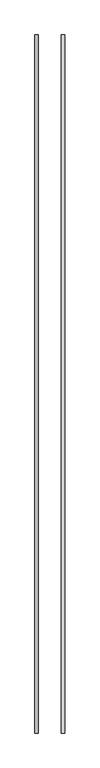
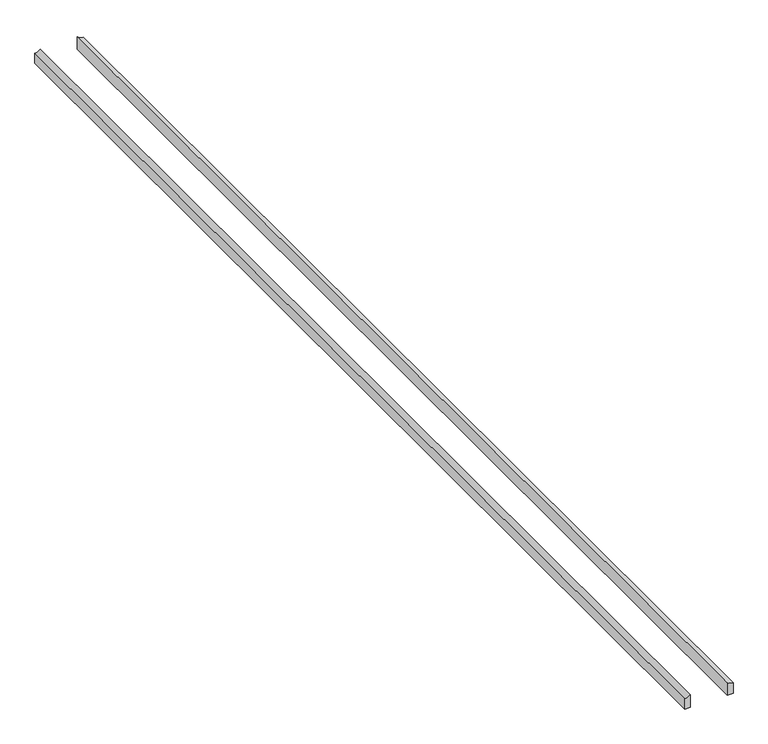
"""IFC4 building model written with IfcOpenShell, lengths in millimetres: proxy geometry, Joint027 17850 : Joint027 17850."""

from ifc_helpers import new_model, si_unit, point, frame, frame_2d, origin, place, context, project, spatial, polyline, circle_curve, trimmed, segment, composite_curve, outline, extrude, source, transform, mapped, element, save


def generic_models_950220de(model_context):
    return source(origin(), model_context, "Body", "SweptSolid", [
        extrude(outline(composite_curve([segment(polyline([(40150.796, 7291.9824219), (40131.746, 7291.9824219), (40131.746, 7301.4512927), (40155.1385809, 7301.4512927)]), True, "CONTINUOUS"), segment(trimmed(circle_curve(frame_2d((40161.3798693, 7292.8587095)), 10.6200833), [point((40155.1385809, 7301.4512927))], [point((40150.796, 7291.9824219))], True, "CARTESIAN"), True, "CONTINUOUS")], self_intersect=False)), frame((0.0, -3747.9491938, 0.0), z_axis=(0.0, 1.0, 0.0), x_axis=(0.0, 0.0, 1.0)), (0.0, 0.0, 1.0), 2000.0),
        extrude(outline(composite_curve([segment(trimmed(circle_curve(frame_2d((40167.1736286, 7377.7892228)), 16.1957742), [point((40150.9781799, 7377.6865442))], [point((40155.1385809, 7366.9512927))], True, "CARTESIAN"), True, "CONTINUOUS"), segment(polyline([(40155.1385809, 7366.9512927), (40131.746, 7366.9512927), (40131.746, 7377.6865442), (40150.9781799, 7377.6865442)]), True, "CONTINUOUS")], self_intersect=False)), frame((0.0, -3747.9491938, 0.0), z_axis=(0.0, 1.0, 0.0), x_axis=(0.0, 0.0, 1.0)), (0.0, 0.0, 1.0), 2000.0),
    ])


if __name__ == "__main__":
    model = new_model("IFC4")
    model_context = context("Model", 3, world=origin())
    ifc_project = project(units=[si_unit("LENGTHUNIT", "METRE", prefix="MILLI")], contexts=[model_context])
    site = spatial("IfcSite", under=ifc_project)
    building = spatial("IfcBuilding", under=site)
    placement = place(None, origin())
    generic_models_shape = generic_models_950220de(model_context)
    element("IfcBuildingElementProxy", 1, Name="Joint027 17850 : Joint027 17850", ObjectType="Joint027 17850 : Joint027 17850", at=placement, inside=building, context=model_context, shape_type="MappedRepresentation", body=[
        mapped(generic_models_shape, transform((0.0, 0.0, 0.0), x_axis=(1.0, 0.0, 0.0), y_axis=(0.0, 1.0, 0.0), z_axis=(0.0, 0.0, 1.0))),
    ])
    save(model, "model.ifc")

# Revit data of these elements
# Type "Joint027 17850 : Joint027 17850"
#   NameOverride = "Joint027"
# Element 1 (IfcBuildingElementProxy, "Joint027 17850 : Joint027 17850")
#   Materials on its faces: "SEALANT"
# Materials
#   "SEALANT": class "Unassigned", colour RGB 142 225 148, transparency 0
